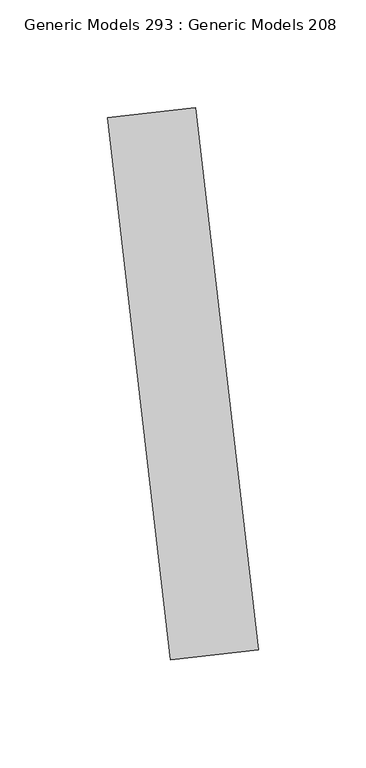
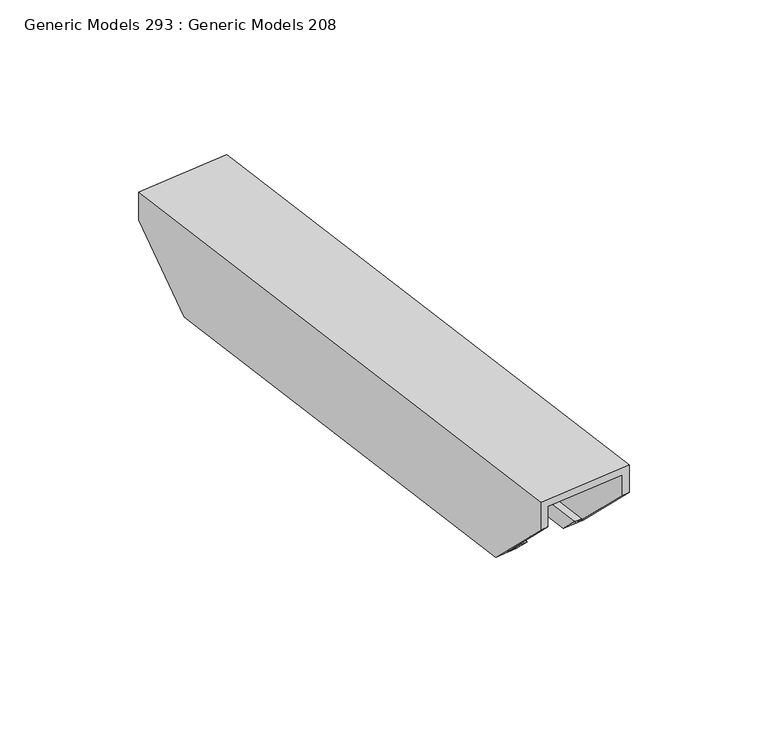
"""IFC4 building model written with IfcOpenShell, lengths in millimetres: proxy geometry, Generic Models 293 : Generic Models 208."""

import ifcopenshell
import ifcopenshell.guid

model = None  # the IFC model being written
_history = None  # IfcOwnerHistory: only IFC2X3 demands one
_inside = {}  # id of a spatial element -> (the spatial element, [elements in it])
_under = {}  # id of a project, library or spatial element -> (it, [spatial elements below it])
_declared = {}  # id of a project -> (the project, [libraries it declares])
_typed = {}  # id of a type object -> (the type object, [elements of that type])
_made_of = {}  # id of a material, layer set ... -> (it, [elements and type objects made of it])


def new_model(schema):
    """Start an empty IFC model of exactly this schema.

    Asked for "IFC4X3", IfcOpenShell would pick the latest addendum, in which some entities
    have other attributes; the version numbers below select the first issue.
    IFC2X3 requires an IfcOwnerHistory on every rooted entity: one is made here for all.
    """
    global model, _history
    if schema == "IFC4X3":
        model = ifcopenshell.file(schema_version=(4, 3, 0, 0))
    else:
        model = ifcopenshell.file(schema=schema)
    _inside.clear()
    _under.clear()
    _declared.clear()
    _typed.clear()
    _made_of.clear()
    _history = None
    if model.schema == "IFC2X3":
        org = make("IfcOrganization", Name="unknown")
        user = make(
            "IfcPersonAndOrganization",
            ThePerson=make("IfcPerson", FamilyName="unknown"),
            TheOrganization=org,
        )
        app = make(
            "IfcApplication",
            ApplicationDeveloper=org,
            Version="unknown",
            ApplicationFullName="unknown",
            ApplicationIdentifier="unknown",
        )
        _history = make(
            "IfcOwnerHistory",
            OwningUser=user,
            OwningApplication=app,
            ChangeAction="ADDED",
            CreationDate=0,
        )
    return model


def make(cls, **values):
    """One entity of the class cls with the attributes given. An attribute that is None is left unset."""
    return model.create_entity(
        cls, **{name: value for name, value in values.items() if value is not None}
    )


def rooted(cls, **values):
    """An entity with a GlobalId (a new one), such as an element, a storey or a relation."""
    return make(cls, GlobalId=ifcopenshell.guid.new(), OwnerHistory=_history, **values)


def si_unit(unit_type, name, prefix=None):
    """IfcSIUnit, for example si_unit("LENGTHUNIT", "METRE", prefix="MILLI")."""
    return make("IfcSIUnit", UnitType=unit_type, Prefix=prefix, Name=name)


def assignment(units):
    """IfcUnitAssignment: the units of a project."""
    return None if units is None else make("IfcUnitAssignment", Units=units)


def point(xyz):
    """IfcCartesianPoint."""
    return None if xyz is None else make("IfcCartesianPoint", Coordinates=xyz)


def direction(xyz):
    """IfcDirection."""
    return None if xyz is None else make("IfcDirection", DirectionRatios=xyz)


def frame(location, z_axis=None, x_axis=None):
    """IfcAxis2Placement3D, a coordinate frame: its origin and axes. An axis left out is left unset."""
    return make(
        "IfcAxis2Placement3D",
        Location=point(location),
        Axis=direction(z_axis),
        RefDirection=direction(x_axis),
    )


def origin():
    """The frame at (0, 0, 0) with its axes left unset."""
    return frame((0.0, 0.0, 0.0))


def place(relative_to, where):
    """IfcLocalPlacement: puts the frame where relative to a parent placement (None: the world)."""
    return make(
        "IfcLocalPlacement", PlacementRelTo=relative_to, RelativePlacement=where
    )


def context(
    kind, dimensions, precision=None, world=None, true_north=None, identifier=None
):
    """IfcGeometricRepresentationContext, for example the 3D "Model" context."""
    return make(
        "IfcGeometricRepresentationContext",
        ContextIdentifier=identifier,
        ContextType=kind,
        CoordinateSpaceDimension=dimensions,
        Precision=precision,
        WorldCoordinateSystem=world,
        TrueNorth=true_north,
    )


def project(units=None, contexts=None):
    """IfcProject with its units and contexts."""
    return rooted(
        "IfcProject",
        Name="project",
        RepresentationContexts=contexts,
        UnitsInContext=assignment(units),
    )


def spatial(cls, under=None, at=None, **own):
    """A site, building, storey or space (cls), placed at a placement, below another one or the project."""
    s = rooted(cls, ObjectPlacement=at, **own)
    if under is not None:
        _under.setdefault(under.id(), (under, []))[1].append(s)
    return s


def faces_of(points, faces, orient=None, outer=None):
    """IfcFace entities. A face is a list of loops; a loop is a list of indices into points, from 0.

    orient and outer hold one flag for each loop. By default every Orientation is true, the
    first loop of a face is its IfcFaceOuterBound and the others are IfcFaceBound.
    """
    made = []
    for i, loops in enumerate(faces):
        bounds = []
        for j, loop in enumerate(loops):
            is_outer = j == 0 if outer is None else outer[i][j]
            bounds.append(
                make(
                    "IfcFaceOuterBound" if is_outer else "IfcFaceBound",
                    Bound=make("IfcPolyLoop", Polygon=[points[k] for k in loop]),
                    Orientation=True if orient is None else orient[i][j],
                )
            )
        made.append(make("IfcFace", Bounds=bounds))
    return made


def faceted_brep(points, faces, orient=None, outer=None, voids=None):
    """IfcFacetedBrep: a solid bounded by flat faces; with voids (closed shells), ...WithVoids."""
    shared = [point(p) for p in points]
    hull = make("IfcClosedShell", CfsFaces=faces_of(shared, faces, orient, outer))
    if voids is None:
        return make("IfcFacetedBrep", Outer=hull)
    return make(
        "IfcFacetedBrepWithVoids",
        Outer=hull,
        Voids=[
            make(cls, CfsFaces=faces_of(shared, fs, o, b)) for cls, fs, o, b in voids
        ],
    )


def shape(context_of_items, identifier, shape_type, items):
    """IfcShapeRepresentation: the items that make up one representation, for example the "Body"."""
    return make(
        "IfcShapeRepresentation",
        ContextOfItems=context_of_items,
        RepresentationIdentifier=identifier,
        RepresentationType=shape_type,
        Items=items,
    )


def source(mapping_origin, context_of_items, identifier, shape_type, items):
    """IfcRepresentationMap: a shape defined once, which mapped items show again and again."""
    return make(
        "IfcRepresentationMap",
        MappingOrigin=mapping_origin,
        MappedRepresentation=shape(context_of_items, identifier, shape_type, items),
    )


def transform(
    local_origin,
    x_axis=None,
    y_axis=None,
    z_axis=None,
    scale=None,
    scale2=None,
    scale3=None,
    uniform=True,
):
    """IfcCartesianTransformationOperator3D, or its non-uniform kind. x_axis, y_axis, z_axis: its Axis1, 2, 3."""
    if uniform:
        return make(
            "IfcCartesianTransformationOperator3D",
            Axis1=direction(x_axis),
            Axis2=direction(y_axis),
            LocalOrigin=point(local_origin),
            Scale=scale,
            Axis3=direction(z_axis),
        )
    return make(
        "IfcCartesianTransformationOperator3DnonUniform",
        Axis1=direction(x_axis),
        Axis2=direction(y_axis),
        LocalOrigin=point(local_origin),
        Scale=scale,
        Axis3=direction(z_axis),
        Scale2=scale2,
        Scale3=scale3,
    )


def mapped(mapping_source, mapping_target):
    """IfcMappedItem: shows the shape of a source again, moved by a transform."""
    return make(
        "IfcMappedItem", MappingSource=mapping_source, MappingTarget=mapping_target
    )


def made_of(thing, what):
    """Note that an element or type object is made of a material, layer set ...; save() writes the relation."""
    if what is not None:
        _made_of.setdefault(what.id(), (what, []))[1].append(thing)
    return thing


def element(
    cls,
    number,
    at=None,
    inside=None,
    cuts=None,
    type_object=None,
    material=None,
    context=None,
    identifier="Body",
    shape_type=None,
    held_by="IfcProductDefinitionShape",
    body=None,
    shapes=None,
    **own,
):
    """One element of the class cls, such as IfcWall. Its Tag is "e" and its number.

    at: its placement. inside: the storey or other place that contains it. cuts: it is an
    opening in that element (IfcRelVoidsElement). A single representation is given by context,
    identifier, shape_type and body (its items); several are given by shapes. held_by: the class
    of the entity that holds the representations. save() writes the other relations.
    """
    e = rooted(cls, Tag="e%d" % number, ObjectPlacement=at, **own)
    if body is not None:
        shapes = [shape(context, identifier, shape_type, body)]
    if shapes is not None:
        e.Representation = make(held_by, Representations=shapes)
    if inside is not None:
        _inside.setdefault(inside.id(), (inside, []))[1].append(e)
    if cuts is not None:
        rooted(
            "IfcRelVoidsElement", RelatingBuildingElement=cuts, RelatedOpeningElement=e
        )
    if type_object is not None:
        _typed.setdefault(type_object.id(), (type_object, []))[1].append(e)
    return made_of(e, material)


def aggregate(whole, parts):
    """IfcRelAggregates: a whole, such as a stair, and the parts it consists of."""
    return rooted("IfcRelAggregates", RelatingObject=whole, RelatedObjects=parts)


def save(model, path):
    """Write the relations noted so far, then the file.

    IfcRelAggregates (storeys below a building ...), IfcRelContainedInSpatialStructure (elements
    in a storey), IfcRelDefinesByType, IfcRelAssociatesMaterial and IfcRelDeclares: one each for
    every whole, place, type object, material and project.
    """
    for whole, parts in _under.values():
        aggregate(whole, parts)
    for where, things in _inside.values():
        rooted(
            "IfcRelContainedInSpatialStructure",
            RelatedElements=things,
            RelatingStructure=where,
        )
    for kind, things in _typed.values():
        rooted("IfcRelDefinesByType", RelatedObjects=things, RelatingType=kind)
    for what, things in _made_of.values():
        rooted("IfcRelAssociatesMaterial", RelatedObjects=things, RelatingMaterial=what)
    for by, libraries in _declared.values():
        rooted("IfcRelDeclares", RelatingContext=by, RelatedDefinitions=libraries)
    model.write(path)


def generic_models_293_generic_models_208_f168c3c5(model_context):
    return source(origin(), model_context, "Body", "Brep", [
        faceted_brep([(-1209.8976106, -22067.8380575, 1035.05), (-1168.89849, -22063.0738441, 1035.05), (-1168.89849, -22063.0738441, 1022.35), (-1172.0522685, -22063.4403221, 1022.35), (-1172.0522685, -22063.4403221, 1031.875), (-1206.7438321, -22067.4715796, 1031.875), (-1206.7438321, -22067.4715796, 1022.35), (-1209.8976106, -22067.8380575, 1022.35), (-1177.4255958, -22319.7738606, 1031.875), (-1142.7340321, -22315.7426031, 1031.875), (-1142.7340321, -22315.7426031, 1022.35), (-1139.5802536, -22315.3761252, 1022.35), (-1139.5802536, -22315.3761252, 1035.05), (-1180.5793743, -22320.1403386, 1035.05), (-1180.5793743, -22320.1403386, 1022.35), (-1177.4255958, -22319.7738606, 1022.35), (-1142.8785552, -22286.9921185, 993.775), (-1165.6001884, -22091.4578507, 993.775), (-1169.1204448, -22088.6705502, 996.95), (-1145.6658558, -22290.512375, 996.95), (-1172.2742234, -22089.0370281, 996.95), (-1148.8196343, -22290.878853, 996.95), (-1172.7323208, -22085.094805, 1000.91875), (-1148.3615368, -22294.8210761, 1000.91875), (-1175.8860993, -22085.4612829, 1000.91875), (-1151.5153154, -22295.1875541, 1000.91875), (-1175.0615239, -22092.5572846, 993.775), (-1152.3398908, -22288.0915524, 993.775), (-1206.599309, -22096.2220641, 993.775), (-1183.8776759, -22291.7563319, 993.775), (-1197.1379735, -22095.1226303, 993.775), (-1174.4163404, -22290.6568981, 993.775), (-1197.9625489, -22088.0266286, 1000.91875), (-1173.591765, -22297.7528997, 1000.91875), (-1201.1163274, -22088.3931066, 1000.91875), (-1176.7455435, -22298.1193777, 1000.91875), (-1200.65823, -22092.3353297, 996.95), (-1177.2036409, -22294.1771546, 996.95), (-1203.8120085, -22092.7018077, 996.95), (-1180.3574194, -22294.5436325, 996.95)], [[[0, 1, 2, 3, 4, 5, 6, 7]], [[8, 9, 10, 11, 12, 13, 14, 15]], [[5, 4, 9, 8]], [[1, 12, 11, 16, 17, 2]], [[1, 0, 13, 12]], [[9, 4, 3, 18, 19, 10]], [[19, 18, 20, 21]], [[21, 20, 22, 23]], [[23, 22, 24, 25]], [[25, 24, 26, 27]], [[27, 26, 17, 16]], [[13, 0, 7, 28, 29, 14]], [[29, 28, 30, 31]], [[31, 30, 32, 33]], [[33, 32, 34, 35]], [[35, 34, 36, 37]], [[37, 36, 38, 39]], [[5, 8, 15, 39, 38, 6]], [[11, 10, 19, 21, 23, 25, 27, 16]], [[15, 14, 29, 31, 33, 35, 37, 39]], [[3, 2, 17, 26, 24, 22, 20, 18]], [[7, 6, 38, 36, 34, 32, 30, 28]]]),
    ])


if __name__ == "__main__":
    model = new_model("IFC4")
    model_context = context("Model", 3, world=origin())
    ifc_project = project(units=[si_unit("LENGTHUNIT", "METRE", prefix="MILLI")], contexts=[model_context])
    site = spatial("IfcSite", under=ifc_project)
    building = spatial("IfcBuilding", under=site)
    placement = place(None, origin())
    generic_models_293_generic_models_208_shape = generic_models_293_generic_models_208_f168c3c5(model_context)
    element("IfcBuildingElementProxy", 1, Name="Generic Models 293 : Generic Models 208", ObjectType="Generic Models 293 : Generic Models 208", at=placement, inside=building, context=model_context, shape_type="MappedRepresentation", body=[
        mapped(generic_models_293_generic_models_208_shape, transform((0.0, 0.0, 0.0), x_axis=(1.0, 0.0, 0.0), y_axis=(0.0, 1.0, 0.0), z_axis=(0.0, 0.0, 1.0))),
    ])
    save(model, "model.ifc")

# Revit data of these elements
# Element 1 (IfcBuildingElementProxy, "Generic Models 293 : Generic Models 208")
#   Materials on its faces: "UNISTRUT P1000, 1 5/8\" X 1 5/8\", CHANNEL OR ALUM. CHANNEL"
# Materials
#   "UNISTRUT P1000, 1 5/8\" X 1 5/8\", CHANNEL OR ALUM. CHANNEL": class "Metal", colour RGB 244 244 244, transparency 0, Description = "Aluminum 6061", Cost = 0
